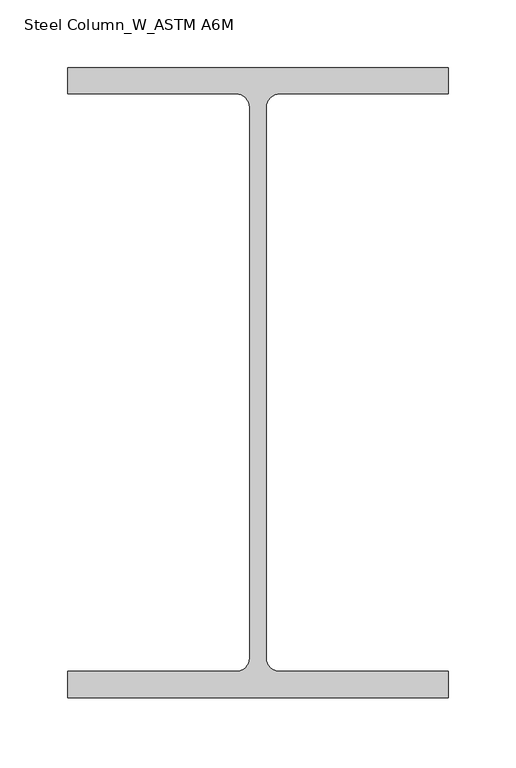
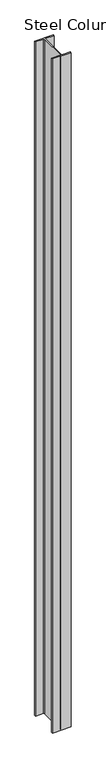
"""IFC4 building model written with IfcOpenShell, lengths in millimetres: column geometry, Steel Column_W_ASTM A6M : H_SC_AR_S01_W460x128_C1."""

import ifcopenshell
import ifcopenshell.guid

model = None  # the IFC model being written
_history = None  # IfcOwnerHistory: only IFC2X3 demands one
_inside = {}  # id of a spatial element -> (the spatial element, [elements in it])
_under = {}  # id of a project, library or spatial element -> (it, [spatial elements below it])
_declared = {}  # id of a project -> (the project, [libraries it declares])
_typed = {}  # id of a type object -> (the type object, [elements of that type])
_made_of = {}  # id of a material, layer set ... -> (it, [elements and type objects made of it])


def new_model(schema):
    """Start an empty IFC model of exactly this schema.

    Asked for "IFC4X3", IfcOpenShell would pick the latest addendum, in which some entities
    have other attributes; the version numbers below select the first issue.
    IFC2X3 requires an IfcOwnerHistory on every rooted entity: one is made here for all.
    """
    global model, _history
    if schema == "IFC4X3":
        model = ifcopenshell.file(schema_version=(4, 3, 0, 0))
    else:
        model = ifcopenshell.file(schema=schema)
    _inside.clear()
    _under.clear()
    _declared.clear()
    _typed.clear()
    _made_of.clear()
    _history = None
    if model.schema == "IFC2X3":
        org = make("IfcOrganization", Name="unknown")
        user = make(
            "IfcPersonAndOrganization",
            ThePerson=make("IfcPerson", FamilyName="unknown"),
            TheOrganization=org,
        )
        app = make(
            "IfcApplication",
            ApplicationDeveloper=org,
            Version="unknown",
            ApplicationFullName="unknown",
            ApplicationIdentifier="unknown",
        )
        _history = make(
            "IfcOwnerHistory",
            OwningUser=user,
            OwningApplication=app,
            ChangeAction="ADDED",
            CreationDate=0,
        )
    return model


def make(cls, **values):
    """One entity of the class cls with the attributes given. An attribute that is None is left unset."""
    return model.create_entity(
        cls, **{name: value for name, value in values.items() if value is not None}
    )


def rooted(cls, **values):
    """An entity with a GlobalId (a new one), such as an element, a storey or a relation."""
    return make(cls, GlobalId=ifcopenshell.guid.new(), OwnerHistory=_history, **values)


def si_unit(unit_type, name, prefix=None):
    """IfcSIUnit, for example si_unit("LENGTHUNIT", "METRE", prefix="MILLI")."""
    return make("IfcSIUnit", UnitType=unit_type, Prefix=prefix, Name=name)


def assignment(units):
    """IfcUnitAssignment: the units of a project."""
    return None if units is None else make("IfcUnitAssignment", Units=units)


def point(xyz):
    """IfcCartesianPoint."""
    return None if xyz is None else make("IfcCartesianPoint", Coordinates=xyz)


def direction(xyz):
    """IfcDirection."""
    return None if xyz is None else make("IfcDirection", DirectionRatios=xyz)


def frame(location, z_axis=None, x_axis=None):
    """IfcAxis2Placement3D, a coordinate frame: its origin and axes. An axis left out is left unset."""
    return make(
        "IfcAxis2Placement3D",
        Location=point(location),
        Axis=direction(z_axis),
        RefDirection=direction(x_axis),
    )


def frame_2d(location, x_axis=None):
    """IfcAxis2Placement2D, a coordinate frame in the plane: its origin and x axis."""
    return make(
        "IfcAxis2Placement2D", Location=point(location), RefDirection=direction(x_axis)
    )


def origin():
    """The frame at (0, 0, 0) with its axes left unset."""
    return frame((0.0, 0.0, 0.0))


def place(relative_to, where):
    """IfcLocalPlacement: puts the frame where relative to a parent placement (None: the world)."""
    return make(
        "IfcLocalPlacement", PlacementRelTo=relative_to, RelativePlacement=where
    )


def context(
    kind, dimensions, precision=None, world=None, true_north=None, identifier=None
):
    """IfcGeometricRepresentationContext, for example the 3D "Model" context."""
    return make(
        "IfcGeometricRepresentationContext",
        ContextIdentifier=identifier,
        ContextType=kind,
        CoordinateSpaceDimension=dimensions,
        Precision=precision,
        WorldCoordinateSystem=world,
        TrueNorth=true_north,
    )


def project(units=None, contexts=None):
    """IfcProject with its units and contexts."""
    return rooted(
        "IfcProject",
        Name="project",
        RepresentationContexts=contexts,
        UnitsInContext=assignment(units),
    )


def spatial(cls, under=None, at=None, **own):
    """A site, building, storey or space (cls), placed at a placement, below another one or the project."""
    s = rooted(cls, ObjectPlacement=at, **own)
    if under is not None:
        _under.setdefault(under.id(), (under, []))[1].append(s)
    return s


def polyline(points):
    """IfcPolyline through the points."""
    return make("IfcPolyline", Points=[point(p) for p in points])


def circle_curve(where, radius):
    """IfcCircle in the frame where."""
    return make("IfcCircle", Position=where, Radius=radius)


def trimmed(basis, trim1, trim2, sense, master):
    """IfcTrimmedCurve: the piece of a basis curve between two trims."""
    return make(
        "IfcTrimmedCurve",
        BasisCurve=basis,
        Trim1=trim1,
        Trim2=trim2,
        SenseAgreement=sense,
        MasterRepresentation=master,
    )


def segment(curve, same_sense, transition):
    """IfcCompositeCurveSegment."""
    return make(
        "IfcCompositeCurveSegment",
        Transition=transition,
        SameSense=same_sense,
        ParentCurve=curve,
    )


def composite_curve(segments, self_intersect=None):
    """IfcCompositeCurve: segments joined end to end."""
    return make("IfcCompositeCurve", Segments=segments, SelfIntersect=self_intersect)


def outline(outer, holes=None, kind="AREA"):
    """IfcArbitraryClosedProfileDef: a profile drawn as a closed curve; with holes, ...WithVoids."""
    if holes is None:
        return make("IfcArbitraryClosedProfileDef", ProfileType=kind, OuterCurve=outer)
    return make(
        "IfcArbitraryProfileDefWithVoids",
        ProfileType=kind,
        OuterCurve=outer,
        InnerCurves=holes,
    )


def extrude(swept, where, along, depth):
    """IfcExtrudedAreaSolid: the profile swept, set in the frame where, extruded along a direction by depth."""
    return make(
        "IfcExtrudedAreaSolid",
        SweptArea=swept,
        Position=where,
        ExtrudedDirection=direction(along),
        Depth=depth,
    )


def shape(context_of_items, identifier, shape_type, items):
    """IfcShapeRepresentation: the items that make up one representation, for example the "Body"."""
    return make(
        "IfcShapeRepresentation",
        ContextOfItems=context_of_items,
        RepresentationIdentifier=identifier,
        RepresentationType=shape_type,
        Items=items,
    )


def source(mapping_origin, context_of_items, identifier, shape_type, items):
    """IfcRepresentationMap: a shape defined once, which mapped items show again and again."""
    return make(
        "IfcRepresentationMap",
        MappingOrigin=mapping_origin,
        MappedRepresentation=shape(context_of_items, identifier, shape_type, items),
    )


def transform(
    local_origin,
    x_axis=None,
    y_axis=None,
    z_axis=None,
    scale=None,
    scale2=None,
    scale3=None,
    uniform=True,
):
    """IfcCartesianTransformationOperator3D, or its non-uniform kind. x_axis, y_axis, z_axis: its Axis1, 2, 3."""
    if uniform:
        return make(
            "IfcCartesianTransformationOperator3D",
            Axis1=direction(x_axis),
            Axis2=direction(y_axis),
            LocalOrigin=point(local_origin),
            Scale=scale,
            Axis3=direction(z_axis),
        )
    return make(
        "IfcCartesianTransformationOperator3DnonUniform",
        Axis1=direction(x_axis),
        Axis2=direction(y_axis),
        LocalOrigin=point(local_origin),
        Scale=scale,
        Axis3=direction(z_axis),
        Scale2=scale2,
        Scale3=scale3,
    )


def mapped(mapping_source, mapping_target):
    """IfcMappedItem: shows the shape of a source again, moved by a transform."""
    return make(
        "IfcMappedItem", MappingSource=mapping_source, MappingTarget=mapping_target
    )


def made_of(thing, what):
    """Note that an element or type object is made of a material, layer set ...; save() writes the relation."""
    if what is not None:
        _made_of.setdefault(what.id(), (what, []))[1].append(thing)
    return thing


def element(
    cls,
    number,
    at=None,
    inside=None,
    cuts=None,
    type_object=None,
    material=None,
    context=None,
    identifier="Body",
    shape_type=None,
    held_by="IfcProductDefinitionShape",
    body=None,
    shapes=None,
    **own,
):
    """One element of the class cls, such as IfcWall. Its Tag is "e" and its number.

    at: its placement. inside: the storey or other place that contains it. cuts: it is an
    opening in that element (IfcRelVoidsElement). A single representation is given by context,
    identifier, shape_type and body (its items); several are given by shapes. held_by: the class
    of the entity that holds the representations. save() writes the other relations.
    """
    e = rooted(cls, Tag="e%d" % number, ObjectPlacement=at, **own)
    if body is not None:
        shapes = [shape(context, identifier, shape_type, body)]
    if shapes is not None:
        e.Representation = make(held_by, Representations=shapes)
    if inside is not None:
        _inside.setdefault(inside.id(), (inside, []))[1].append(e)
    if cuts is not None:
        rooted(
            "IfcRelVoidsElement", RelatingBuildingElement=cuts, RelatedOpeningElement=e
        )
    if type_object is not None:
        _typed.setdefault(type_object.id(), (type_object, []))[1].append(e)
    return made_of(e, material)


def aggregate(whole, parts):
    """IfcRelAggregates: a whole, such as a stair, and the parts it consists of."""
    return rooted("IfcRelAggregates", RelatingObject=whole, RelatedObjects=parts)


def save(model, path):
    """Write the relations noted so far, then the file.

    IfcRelAggregates (storeys below a building ...), IfcRelContainedInSpatialStructure (elements
    in a storey), IfcRelDefinesByType, IfcRelAssociatesMaterial and IfcRelDeclares: one each for
    every whole, place, type object, material and project.
    """
    for whole, parts in _under.values():
        aggregate(whole, parts)
    for where, things in _inside.values():
        rooted(
            "IfcRelContainedInSpatialStructure",
            RelatedElements=things,
            RelatingStructure=where,
        )
    for kind, things in _typed.values():
        rooted("IfcRelDefinesByType", RelatedObjects=things, RelatingType=kind)
    for what, things in _made_of.values():
        rooted("IfcRelAssociatesMaterial", RelatedObjects=things, RelatingMaterial=what)
    for by, libraries in _declared.values():
        rooted("IfcRelDeclares", RelatingContext=by, RelatedDefinitions=libraries)
    model.write(path)


def steel_column_w_astm_a6m_c7f0337f(model_context):
    return source(origin(), model_context, "Body", "SweptSolid", [
        extrude(outline(composite_curve([segment(polyline([(141.0, 233.5), (141.0, 213.9), (16.2, 213.9)]), True, "CONTINUOUS"), segment(trimmed(circle_curve(frame_2d((16.2, 203.8)), 10.1), [point((16.2, 213.9))], [point((6.1, 203.8))], True, "CARTESIAN"), True, "CONTINUOUS"), segment(polyline([(6.1, 203.8), (6.1, -203.8)]), True, "CONTINUOUS"), segment(trimmed(circle_curve(frame_2d((16.2, -203.8)), 10.1), [point((6.1, -203.8))], [point((16.2, -213.9))], True, "CARTESIAN"), True, "CONTINUOUS"), segment(polyline([(16.2, -213.9), (141.0, -213.9), (141.0, -233.5), (-141.0, -233.5), (-141.0, -213.9), (-16.2, -213.9)]), True, "CONTINUOUS"), segment(trimmed(circle_curve(frame_2d((-16.2, -203.8)), 10.1), [point((-16.2, -213.9))], [point((-6.1, -203.8))], True, "CARTESIAN"), True, "CONTINUOUS"), segment(polyline([(-6.1, -203.8), (-6.1, 203.8)]), True, "CONTINUOUS"), segment(trimmed(circle_curve(frame_2d((-16.2, 203.8)), 10.1), [point((-6.1, 203.8))], [point((-16.2, 213.9))], True, "CARTESIAN"), True, "CONTINUOUS"), segment(polyline([(-16.2, 213.9), (-141.0, 213.9), (-141.0, 233.5), (141.0, 233.5)]), True, "CONTINUOUS")], self_intersect=False)), frame((0.0, 0.0, -7269.1756499), z_axis=(0.0, 0.0, 1.0), x_axis=(1.0, 0.0, 0.0)), (0.0, 0.0, 1.0), 10789.0),
    ])


if __name__ == "__main__":
    model = new_model("IFC4")
    model_context = context("Model", 3, world=origin())
    ifc_project = project(units=[si_unit("LENGTHUNIT", "METRE", prefix="MILLI")], contexts=[model_context])
    site = spatial("IfcSite", under=ifc_project)
    building = spatial("IfcBuilding", under=site)
    placement = place(None, origin())
    steel_column_w_astm_a6m_shape = steel_column_w_astm_a6m_c7f0337f(model_context)
    element("IfcColumn", 1, ObjectType="Steel Column_W_ASTM A6M : H_SC_AR_S01_W460x128_C1", at=placement, inside=building, context=model_context, shape_type="MappedRepresentation", body=[
        mapped(steel_column_w_astm_a6m_shape, transform((0.0, 0.0, 0.0), x_axis=(1.0, 0.0, 0.0), y_axis=(0.0, 1.0, 0.0), z_axis=(0.0, 0.0, 1.0))),
    ])
    save(model, "model.ifc")

# Revit data of these elements
# Type "Steel Column_W_ASTM A6M : H_SC_AR_S01_W460x128_C1"
#   Section Name Key = "W18x86"
#   Width = 28.2 cm
#   Web Thickness = 1.22 cm
#   Web Fillet = 1.01 cm
#   Warping Constant = 3650000.0 cm⁶
#   Torsional Moment of Inertia = 171.00 cm⁴
#   Section Area = 163.0 cm²
#   Plastic Modulus weak axis = 793.0 cm³
#   Plastic Modulus strong axis = 3050.0 cm³
#   Perimeter = 2.02 m²/m
#   Nominal Weight = 128.00 kgf/m
#   Moment of Inertia weak axis = 7280.00 cm⁴
#   Moment of Inertia strong axis = 63700.00 cm⁴
#   Height = 46.7 cm
#   Flange Thickness = 1.96 cm
#   Elastic Modulus weak axis = 518.0 cm³
#   Elastic Modulus strong axis = 2720.0 cm³
#   Centroid Vertical = 23.35 cm
#   Centroid Horizontal = 14.1 cm
#   Structural Material [instance default] = Steel, 45-345
#   Bolt Spacing = 0
#   Assembly Code = ""
# Element 1 (IfcColumn, "Steel Column_W_ASTM A6M : H_SC_AR_S01_W460x128_C1")
#   Structural Material = none
# Materials
#   "Steel, 45-345": class "Metal", colour RGB 189 187 185, transparency 0, Description = "Steel 345 MPa", Cost = 0
